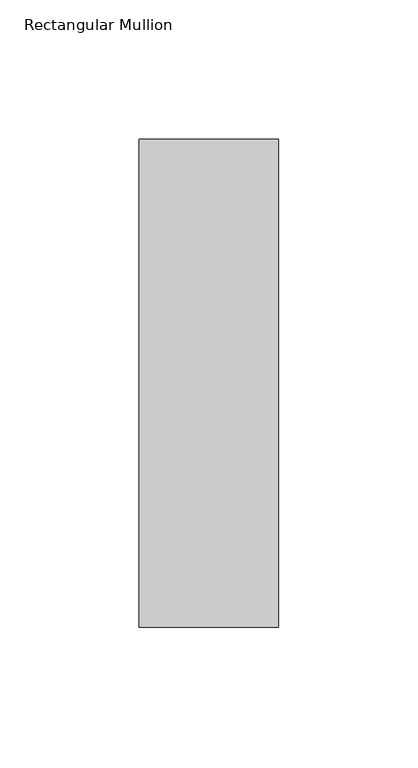
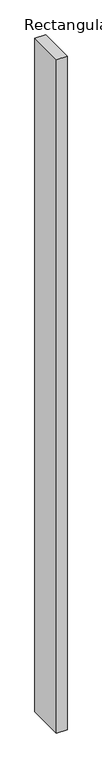
"""IFC4 building model written with IfcOpenShell, lengths in millimetres: member geometry, Rectangular Mullion : WWm-50x175-50mmOffset."""

from ifc_helpers import new_model, si_unit, frame, origin, place, context, project, spatial, polyline, outline, extrude, source, transform, mapped, element, save


def rectangular_mullion_dfe2042f(model_context):
    return source(origin(), model_context, "Body", "SweptSolid", [
        extrude(outline(polyline([(0.0, 87.5), (0.0, -87.5), (-50.0, -87.5), (-50.0, 87.5), (0.0, 87.5)])), frame((0.0, 0.0, -3350.0), z_axis=(0.0, 0.0, 1.0), x_axis=(1.0, 0.0, 0.0)), (0.0, 0.0, 1.0), 3350.0),
    ])


if __name__ == "__main__":
    model = new_model("IFC4")
    model_context = context("Model", 3, world=origin())
    ifc_project = project(units=[si_unit("LENGTHUNIT", "METRE", prefix="MILLI")], contexts=[model_context])
    site = spatial("IfcSite", under=ifc_project)
    building = spatial("IfcBuilding", under=site)
    placement = place(None, origin())
    rectangular_mullion_shape = rectangular_mullion_dfe2042f(model_context)
    element("IfcMember", 1, ObjectType="Rectangular Mullion : WWm-50x175-50mmOffset", at=placement, inside=building, context=model_context, shape_type="MappedRepresentation", body=[
        mapped(rectangular_mullion_shape, transform((0.0, 0.0, 0.0), x_axis=(1.0, 0.0, 0.0), y_axis=(0.0, 1.0, 0.0), z_axis=(0.0, 0.0, 1.0))),
    ])
    save(model, "model.ifc")

# Revit data of these elements
# Type "Rectangular Mullion : WWm-50x175-50mmOffset"
#   built-in parameter 1007304 = 0.574147 (stored number, unit not read)
#   built-in parameter 1007301 = 0.082021 (stored number, unit not read)
#   built-in parameter 1007300 = 0.082021 (stored number, unit not read)
# Element 1 (IfcMember, "Rectangular Mullion : WWm-50x175-50mmOffset")
#   Materials on its faces: "WW-EC-RGB-Mullion"
# Materials
#   "WW-EC-RGB-Mullion": class "Generic", colour RGB 255 255 255, transparency 0, Comments = "If region requests black mullions, switch asset color to RGB 25-25-25", Description = "Generic Color", Cost = 0
